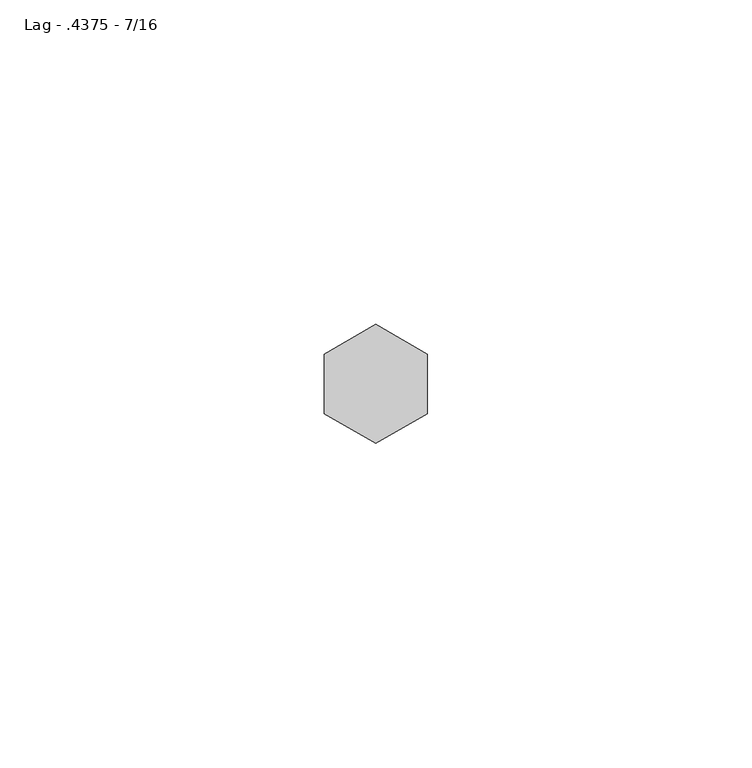
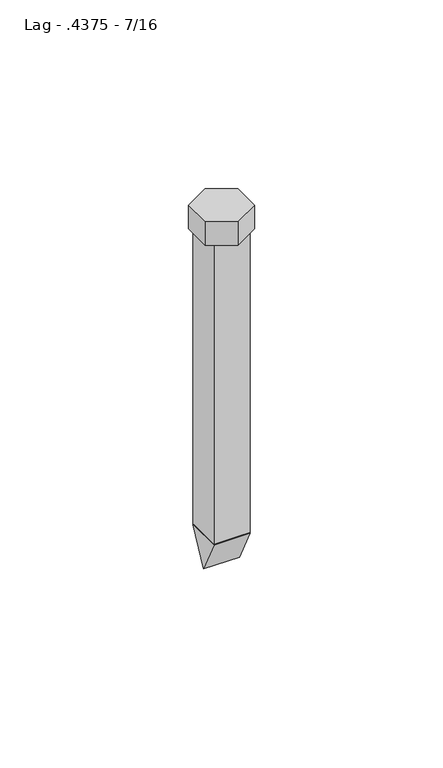
"""IFC4 building model written with IfcOpenShell, lengths in millimetres: fastener geometry, 060523 - W_P_C - Fastenings - Generic - SQUARE : Lag - .4375 - 7/16."""

import ifcopenshell
import ifcopenshell.guid

model = None  # the IFC model being written
_history = None  # IfcOwnerHistory: only IFC2X3 demands one
_inside = {}  # id of a spatial element -> (the spatial element, [elements in it])
_under = {}  # id of a project, library or spatial element -> (it, [spatial elements below it])
_declared = {}  # id of a project -> (the project, [libraries it declares])
_typed = {}  # id of a type object -> (the type object, [elements of that type])
_made_of = {}  # id of a material, layer set ... -> (it, [elements and type objects made of it])


def new_model(schema):
    """Start an empty IFC model of exactly this schema.

    Asked for "IFC4X3", IfcOpenShell would pick the latest addendum, in which some entities
    have other attributes; the version numbers below select the first issue.
    IFC2X3 requires an IfcOwnerHistory on every rooted entity: one is made here for all.
    """
    global model, _history
    if schema == "IFC4X3":
        model = ifcopenshell.file(schema_version=(4, 3, 0, 0))
    else:
        model = ifcopenshell.file(schema=schema)
    _inside.clear()
    _under.clear()
    _declared.clear()
    _typed.clear()
    _made_of.clear()
    _history = None
    if model.schema == "IFC2X3":
        org = make("IfcOrganization", Name="unknown")
        user = make(
            "IfcPersonAndOrganization",
            ThePerson=make("IfcPerson", FamilyName="unknown"),
            TheOrganization=org,
        )
        app = make(
            "IfcApplication",
            ApplicationDeveloper=org,
            Version="unknown",
            ApplicationFullName="unknown",
            ApplicationIdentifier="unknown",
        )
        _history = make(
            "IfcOwnerHistory",
            OwningUser=user,
            OwningApplication=app,
            ChangeAction="ADDED",
            CreationDate=0,
        )
    return model


def make(cls, **values):
    """One entity of the class cls with the attributes given. An attribute that is None is left unset."""
    return model.create_entity(
        cls, **{name: value for name, value in values.items() if value is not None}
    )


def rooted(cls, **values):
    """An entity with a GlobalId (a new one), such as an element, a storey or a relation."""
    return make(cls, GlobalId=ifcopenshell.guid.new(), OwnerHistory=_history, **values)


def si_unit(unit_type, name, prefix=None):
    """IfcSIUnit, for example si_unit("LENGTHUNIT", "METRE", prefix="MILLI")."""
    return make("IfcSIUnit", UnitType=unit_type, Prefix=prefix, Name=name)


def assignment(units):
    """IfcUnitAssignment: the units of a project."""
    return None if units is None else make("IfcUnitAssignment", Units=units)


def point(xyz):
    """IfcCartesianPoint."""
    return None if xyz is None else make("IfcCartesianPoint", Coordinates=xyz)


def direction(xyz):
    """IfcDirection."""
    return None if xyz is None else make("IfcDirection", DirectionRatios=xyz)


def frame(location, z_axis=None, x_axis=None):
    """IfcAxis2Placement3D, a coordinate frame: its origin and axes. An axis left out is left unset."""
    return make(
        "IfcAxis2Placement3D",
        Location=point(location),
        Axis=direction(z_axis),
        RefDirection=direction(x_axis),
    )


def origin():
    """The frame at (0, 0, 0) with its axes left unset."""
    return frame((0.0, 0.0, 0.0))


def origin_with_axes():
    """The frame at (0, 0, 0) with the z axis (0, 0, 1) and the x axis (1, 0, 0) written out."""
    return frame((0.0, 0.0, 0.0), z_axis=(0.0, 0.0, 1.0), x_axis=(1.0, 0.0, 0.0))


def place(relative_to, where):
    """IfcLocalPlacement: puts the frame where relative to a parent placement (None: the world)."""
    return make(
        "IfcLocalPlacement", PlacementRelTo=relative_to, RelativePlacement=where
    )


def context(
    kind, dimensions, precision=None, world=None, true_north=None, identifier=None
):
    """IfcGeometricRepresentationContext, for example the 3D "Model" context."""
    return make(
        "IfcGeometricRepresentationContext",
        ContextIdentifier=identifier,
        ContextType=kind,
        CoordinateSpaceDimension=dimensions,
        Precision=precision,
        WorldCoordinateSystem=world,
        TrueNorth=true_north,
    )


def project(units=None, contexts=None):
    """IfcProject with its units and contexts."""
    return rooted(
        "IfcProject",
        Name="project",
        RepresentationContexts=contexts,
        UnitsInContext=assignment(units),
    )


def spatial(cls, under=None, at=None, **own):
    """A site, building, storey or space (cls), placed at a placement, below another one or the project."""
    s = rooted(cls, ObjectPlacement=at, **own)
    if under is not None:
        _under.setdefault(under.id(), (under, []))[1].append(s)
    return s


def polyline(points):
    """IfcPolyline through the points."""
    return make("IfcPolyline", Points=[point(p) for p in points])


def outline(outer, holes=None, kind="AREA"):
    """IfcArbitraryClosedProfileDef: a profile drawn as a closed curve; with holes, ...WithVoids."""
    if holes is None:
        return make("IfcArbitraryClosedProfileDef", ProfileType=kind, OuterCurve=outer)
    return make(
        "IfcArbitraryProfileDefWithVoids",
        ProfileType=kind,
        OuterCurve=outer,
        InnerCurves=holes,
    )


def extrude(swept, where, along, depth):
    """IfcExtrudedAreaSolid: the profile swept, set in the frame where, extruded along a direction by depth."""
    return make(
        "IfcExtrudedAreaSolid",
        SweptArea=swept,
        Position=where,
        ExtrudedDirection=direction(along),
        Depth=depth,
    )


def shape(context_of_items, identifier, shape_type, items):
    """IfcShapeRepresentation: the items that make up one representation, for example the "Body"."""
    return make(
        "IfcShapeRepresentation",
        ContextOfItems=context_of_items,
        RepresentationIdentifier=identifier,
        RepresentationType=shape_type,
        Items=items,
    )


def source(mapping_origin, context_of_items, identifier, shape_type, items):
    """IfcRepresentationMap: a shape defined once, which mapped items show again and again."""
    return make(
        "IfcRepresentationMap",
        MappingOrigin=mapping_origin,
        MappedRepresentation=shape(context_of_items, identifier, shape_type, items),
    )


def transform(
    local_origin,
    x_axis=None,
    y_axis=None,
    z_axis=None,
    scale=None,
    scale2=None,
    scale3=None,
    uniform=True,
):
    """IfcCartesianTransformationOperator3D, or its non-uniform kind. x_axis, y_axis, z_axis: its Axis1, 2, 3."""
    if uniform:
        return make(
            "IfcCartesianTransformationOperator3D",
            Axis1=direction(x_axis),
            Axis2=direction(y_axis),
            LocalOrigin=point(local_origin),
            Scale=scale,
            Axis3=direction(z_axis),
        )
    return make(
        "IfcCartesianTransformationOperator3DnonUniform",
        Axis1=direction(x_axis),
        Axis2=direction(y_axis),
        LocalOrigin=point(local_origin),
        Scale=scale,
        Axis3=direction(z_axis),
        Scale2=scale2,
        Scale3=scale3,
    )


def mapped(mapping_source, mapping_target):
    """IfcMappedItem: shows the shape of a source again, moved by a transform."""
    return make(
        "IfcMappedItem", MappingSource=mapping_source, MappingTarget=mapping_target
    )


def made_of(thing, what):
    """Note that an element or type object is made of a material, layer set ...; save() writes the relation."""
    if what is not None:
        _made_of.setdefault(what.id(), (what, []))[1].append(thing)
    return thing


def element(
    cls,
    number,
    at=None,
    inside=None,
    cuts=None,
    type_object=None,
    material=None,
    context=None,
    identifier="Body",
    shape_type=None,
    held_by="IfcProductDefinitionShape",
    body=None,
    shapes=None,
    **own,
):
    """One element of the class cls, such as IfcWall. Its Tag is "e" and its number.

    at: its placement. inside: the storey or other place that contains it. cuts: it is an
    opening in that element (IfcRelVoidsElement). A single representation is given by context,
    identifier, shape_type and body (its items); several are given by shapes. held_by: the class
    of the entity that holds the representations. save() writes the other relations.
    """
    e = rooted(cls, Tag="e%d" % number, ObjectPlacement=at, **own)
    if body is not None:
        shapes = [shape(context, identifier, shape_type, body)]
    if shapes is not None:
        e.Representation = make(held_by, Representations=shapes)
    if inside is not None:
        _inside.setdefault(inside.id(), (inside, []))[1].append(e)
    if cuts is not None:
        rooted(
            "IfcRelVoidsElement", RelatingBuildingElement=cuts, RelatedOpeningElement=e
        )
    if type_object is not None:
        _typed.setdefault(type_object.id(), (type_object, []))[1].append(e)
    return made_of(e, material)


def aggregate(whole, parts):
    """IfcRelAggregates: a whole, such as a stair, and the parts it consists of."""
    return rooted("IfcRelAggregates", RelatingObject=whole, RelatedObjects=parts)


def save(model, path):
    """Write the relations noted so far, then the file.

    IfcRelAggregates (storeys below a building ...), IfcRelContainedInSpatialStructure (elements
    in a storey), IfcRelDefinesByType, IfcRelAssociatesMaterial and IfcRelDeclares: one each for
    every whole, place, type object, material and project.
    """
    for whole, parts in _under.values():
        aggregate(whole, parts)
    for where, things in _inside.values():
        rooted(
            "IfcRelContainedInSpatialStructure",
            RelatedElements=things,
            RelatingStructure=where,
        )
    for kind, things in _typed.values():
        rooted("IfcRelDefinesByType", RelatedObjects=things, RelatingType=kind)
    for what, things in _made_of.values():
        rooted("IfcRelAssociatesMaterial", RelatedObjects=things, RelatingMaterial=what)
    for by, libraries in _declared.values():
        rooted("IfcRelDeclares", RelatingContext=by, RelatedDefinitions=libraries)
    model.write(path)


def lag_4375_7_16_16092e99(model_context):
    return source(origin(), model_context, "Body", "SweptSolid", [
        extrude(outline(polyline([(0.0, -113.109375), (-5.7546875, -101.6), (5.7546875, -101.6), (0.0, -113.109375)])), frame((-5.7546875, 0.0, 0.0), z_axis=(1.0, 0.0, 0.0), x_axis=(0.0, 1.0, 0.0)), (0.0, 0.0, 1.0), 11.509375),
        extrude(outline(polyline([(-7.9375, 4.5827178), (0.0, 9.1654355), (7.9375, 4.5827178), (7.9375, -4.5827178), (0.0, -9.1654355), (-7.9375, -4.5827178), (-7.9375, 4.5827178)])), origin_with_axes(), (0.0, 0.0, 1.0), 8.0367187),
        extrude(outline(polyline([(-5.7546875, 5.7546875), (5.7546875, 5.7546875), (5.7546875, -5.7546875), (-5.7546875, -5.7546875), (-5.7546875, 5.7546875)])), frame((0.0, 0.0, -101.6), z_axis=(0.0, 0.0, 1.0), x_axis=(1.0, 0.0, 0.0)), (0.0, 0.0, 1.0), 101.6),
    ])


if __name__ == "__main__":
    model = new_model("IFC4")
    model_context = context("Model", 3, world=origin())
    ifc_project = project(units=[si_unit("LENGTHUNIT", "METRE", prefix="MILLI")], contexts=[model_context])
    site = spatial("IfcSite", under=ifc_project)
    building = spatial("IfcBuilding", under=site)
    placement = place(None, origin())
    lag_4375_7_16_shape = lag_4375_7_16_16092e99(model_context)
    element("IfcFastener", 1, ObjectType="060523 - W_P_C - Fastenings - Generic - SQUARE : Lag - .4375 - 7/16", at=placement, inside=building, context=model_context, shape_type="MappedRepresentation", body=[
        mapped(lag_4375_7_16_shape, transform((0.0, 0.0, 0.0), x_axis=(1.0, 0.0, 0.0), y_axis=(0.0, 1.0, 0.0), z_axis=(0.0, 0.0, 1.0))),
    ])
    save(model, "model.ifc")

# Revit data of these elements
# Type "060523 - W_P_C - Fastenings - Generic - SQUARE : Lag - .4375 - 7/16"
#   Washer_Thickness = 0' - 0 27/256"
#   Washer Radius = 0' - 0 139/256"
#   Washer Offset - Head = 0' - 0"
#   Washer Offset = 0' - 0"
#   Thickness_of_Substrate [instance default] = 0' - 1"
#   Side = 0' - 0.36133"
#   Radius = 0' - 0 29/128"
#   Length [instance default] = 0' - 4"
#   Head Size = 0' - 0 5/8"
#   Head Radius = 0' - 0 5/16"
#   Head Height = 0' - 0 81/256"
#   Double Diameter = 0' - 0 29/32"
#   Diameter = 0' - 0 29/64"
#   Default Elevation = 4' - 0"
#   Washer_Nut_Visibility = no
#   Washer_Head_Visibility = no
#   Round_Head_Visibility = no
#   Point Visibility = yes
#   Nut_Visibility = no
#   Hex_Head_Visiblilty = yes
#   Washer Material = none
#   Bolt Material (Size) = AT SILL - FASTENER AT 24" O.C.
# Element 1 (IfcFastener, "060523 - W_P_C - Fastenings - Generic - SQUARE : Lag - .4375 - 7/16")
#   Materials on its faces: "AT SILL - FASTENER AT 24\" O.C."
# Materials
#   "AT SILL - FASTENER AT 24\" O.C.": class "Generic", colour RGB 120 120 120, transparency 0, Cost = 0
